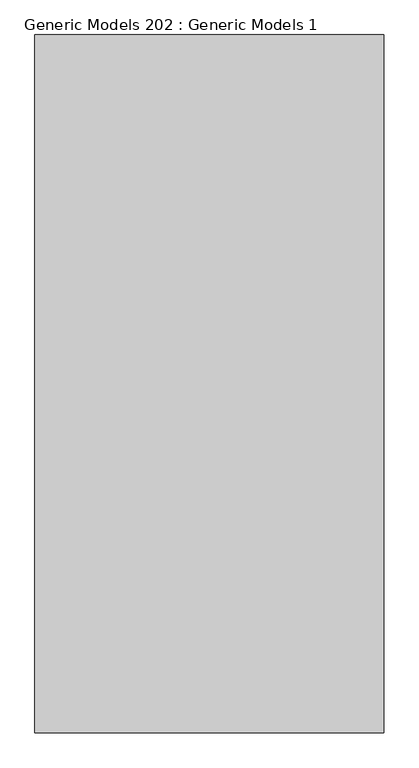
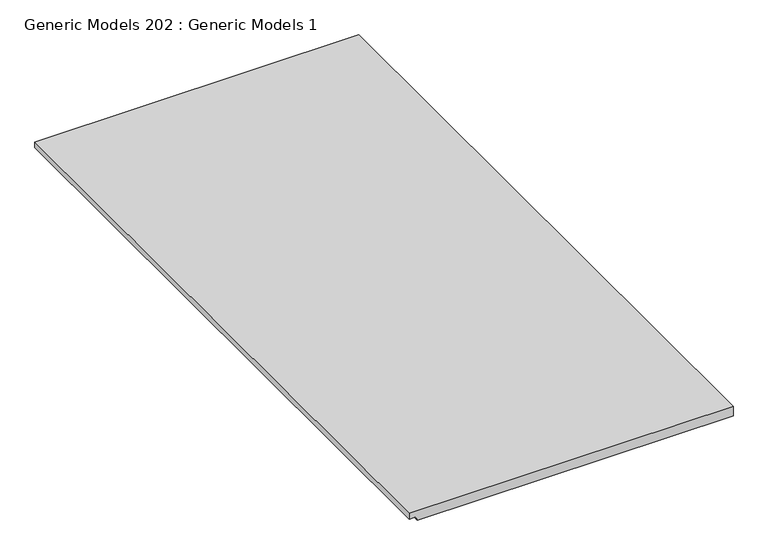
"""IFC4 building model written with IfcOpenShell, lengths in millimetres: proxy geometry, Generic Models 202 : Generic Models 1."""

import ifcopenshell
import ifcopenshell.guid

model = None  # the IFC model being written
_history = None  # IfcOwnerHistory: only IFC2X3 demands one
_inside = {}  # id of a spatial element -> (the spatial element, [elements in it])
_under = {}  # id of a project, library or spatial element -> (it, [spatial elements below it])
_declared = {}  # id of a project -> (the project, [libraries it declares])
_typed = {}  # id of a type object -> (the type object, [elements of that type])
_made_of = {}  # id of a material, layer set ... -> (it, [elements and type objects made of it])


def new_model(schema):
    """Start an empty IFC model of exactly this schema.

    Asked for "IFC4X3", IfcOpenShell would pick the latest addendum, in which some entities
    have other attributes; the version numbers below select the first issue.
    IFC2X3 requires an IfcOwnerHistory on every rooted entity: one is made here for all.
    """
    global model, _history
    if schema == "IFC4X3":
        model = ifcopenshell.file(schema_version=(4, 3, 0, 0))
    else:
        model = ifcopenshell.file(schema=schema)
    _inside.clear()
    _under.clear()
    _declared.clear()
    _typed.clear()
    _made_of.clear()
    _history = None
    if model.schema == "IFC2X3":
        org = make("IfcOrganization", Name="unknown")
        user = make(
            "IfcPersonAndOrganization",
            ThePerson=make("IfcPerson", FamilyName="unknown"),
            TheOrganization=org,
        )
        app = make(
            "IfcApplication",
            ApplicationDeveloper=org,
            Version="unknown",
            ApplicationFullName="unknown",
            ApplicationIdentifier="unknown",
        )
        _history = make(
            "IfcOwnerHistory",
            OwningUser=user,
            OwningApplication=app,
            ChangeAction="ADDED",
            CreationDate=0,
        )
    return model


def make(cls, **values):
    """One entity of the class cls with the attributes given. An attribute that is None is left unset."""
    return model.create_entity(
        cls, **{name: value for name, value in values.items() if value is not None}
    )


def rooted(cls, **values):
    """An entity with a GlobalId (a new one), such as an element, a storey or a relation."""
    return make(cls, GlobalId=ifcopenshell.guid.new(), OwnerHistory=_history, **values)


def si_unit(unit_type, name, prefix=None):
    """IfcSIUnit, for example si_unit("LENGTHUNIT", "METRE", prefix="MILLI")."""
    return make("IfcSIUnit", UnitType=unit_type, Prefix=prefix, Name=name)


def assignment(units):
    """IfcUnitAssignment: the units of a project."""
    return None if units is None else make("IfcUnitAssignment", Units=units)


def point(xyz):
    """IfcCartesianPoint."""
    return None if xyz is None else make("IfcCartesianPoint", Coordinates=xyz)


def direction(xyz):
    """IfcDirection."""
    return None if xyz is None else make("IfcDirection", DirectionRatios=xyz)


def frame(location, z_axis=None, x_axis=None):
    """IfcAxis2Placement3D, a coordinate frame: its origin and axes. An axis left out is left unset."""
    return make(
        "IfcAxis2Placement3D",
        Location=point(location),
        Axis=direction(z_axis),
        RefDirection=direction(x_axis),
    )


def origin():
    """The frame at (0, 0, 0) with its axes left unset."""
    return frame((0.0, 0.0, 0.0))


def place(relative_to, where):
    """IfcLocalPlacement: puts the frame where relative to a parent placement (None: the world)."""
    return make(
        "IfcLocalPlacement", PlacementRelTo=relative_to, RelativePlacement=where
    )


def context(
    kind, dimensions, precision=None, world=None, true_north=None, identifier=None
):
    """IfcGeometricRepresentationContext, for example the 3D "Model" context."""
    return make(
        "IfcGeometricRepresentationContext",
        ContextIdentifier=identifier,
        ContextType=kind,
        CoordinateSpaceDimension=dimensions,
        Precision=precision,
        WorldCoordinateSystem=world,
        TrueNorth=true_north,
    )


def project(units=None, contexts=None):
    """IfcProject with its units and contexts."""
    return rooted(
        "IfcProject",
        Name="project",
        RepresentationContexts=contexts,
        UnitsInContext=assignment(units),
    )


def spatial(cls, under=None, at=None, **own):
    """A site, building, storey or space (cls), placed at a placement, below another one or the project."""
    s = rooted(cls, ObjectPlacement=at, **own)
    if under is not None:
        _under.setdefault(under.id(), (under, []))[1].append(s)
    return s


def polyline(points):
    """IfcPolyline through the points."""
    return make("IfcPolyline", Points=[point(p) for p in points])


def outline(outer, holes=None, kind="AREA"):
    """IfcArbitraryClosedProfileDef: a profile drawn as a closed curve; with holes, ...WithVoids."""
    if holes is None:
        return make("IfcArbitraryClosedProfileDef", ProfileType=kind, OuterCurve=outer)
    return make(
        "IfcArbitraryProfileDefWithVoids",
        ProfileType=kind,
        OuterCurve=outer,
        InnerCurves=holes,
    )


def extrude(swept, where, along, depth):
    """IfcExtrudedAreaSolid: the profile swept, set in the frame where, extruded along a direction by depth."""
    return make(
        "IfcExtrudedAreaSolid",
        SweptArea=swept,
        Position=where,
        ExtrudedDirection=direction(along),
        Depth=depth,
    )


def shape(context_of_items, identifier, shape_type, items):
    """IfcShapeRepresentation: the items that make up one representation, for example the "Body"."""
    return make(
        "IfcShapeRepresentation",
        ContextOfItems=context_of_items,
        RepresentationIdentifier=identifier,
        RepresentationType=shape_type,
        Items=items,
    )


def source(mapping_origin, context_of_items, identifier, shape_type, items):
    """IfcRepresentationMap: a shape defined once, which mapped items show again and again."""
    return make(
        "IfcRepresentationMap",
        MappingOrigin=mapping_origin,
        MappedRepresentation=shape(context_of_items, identifier, shape_type, items),
    )


def transform(
    local_origin,
    x_axis=None,
    y_axis=None,
    z_axis=None,
    scale=None,
    scale2=None,
    scale3=None,
    uniform=True,
):
    """IfcCartesianTransformationOperator3D, or its non-uniform kind. x_axis, y_axis, z_axis: its Axis1, 2, 3."""
    if uniform:
        return make(
            "IfcCartesianTransformationOperator3D",
            Axis1=direction(x_axis),
            Axis2=direction(y_axis),
            LocalOrigin=point(local_origin),
            Scale=scale,
            Axis3=direction(z_axis),
        )
    return make(
        "IfcCartesianTransformationOperator3DnonUniform",
        Axis1=direction(x_axis),
        Axis2=direction(y_axis),
        LocalOrigin=point(local_origin),
        Scale=scale,
        Axis3=direction(z_axis),
        Scale2=scale2,
        Scale3=scale3,
    )


def mapped(mapping_source, mapping_target):
    """IfcMappedItem: shows the shape of a source again, moved by a transform."""
    return make(
        "IfcMappedItem", MappingSource=mapping_source, MappingTarget=mapping_target
    )


def made_of(thing, what):
    """Note that an element or type object is made of a material, layer set ...; save() writes the relation."""
    if what is not None:
        _made_of.setdefault(what.id(), (what, []))[1].append(thing)
    return thing


def element(
    cls,
    number,
    at=None,
    inside=None,
    cuts=None,
    type_object=None,
    material=None,
    context=None,
    identifier="Body",
    shape_type=None,
    held_by="IfcProductDefinitionShape",
    body=None,
    shapes=None,
    **own,
):
    """One element of the class cls, such as IfcWall. Its Tag is "e" and its number.

    at: its placement. inside: the storey or other place that contains it. cuts: it is an
    opening in that element (IfcRelVoidsElement). A single representation is given by context,
    identifier, shape_type and body (its items); several are given by shapes. held_by: the class
    of the entity that holds the representations. save() writes the other relations.
    """
    e = rooted(cls, Tag="e%d" % number, ObjectPlacement=at, **own)
    if body is not None:
        shapes = [shape(context, identifier, shape_type, body)]
    if shapes is not None:
        e.Representation = make(held_by, Representations=shapes)
    if inside is not None:
        _inside.setdefault(inside.id(), (inside, []))[1].append(e)
    if cuts is not None:
        rooted(
            "IfcRelVoidsElement", RelatingBuildingElement=cuts, RelatedOpeningElement=e
        )
    if type_object is not None:
        _typed.setdefault(type_object.id(), (type_object, []))[1].append(e)
    return made_of(e, material)


def aggregate(whole, parts):
    """IfcRelAggregates: a whole, such as a stair, and the parts it consists of."""
    return rooted("IfcRelAggregates", RelatingObject=whole, RelatedObjects=parts)


def save(model, path):
    """Write the relations noted so far, then the file.

    IfcRelAggregates (storeys below a building ...), IfcRelContainedInSpatialStructure (elements
    in a storey), IfcRelDefinesByType, IfcRelAssociatesMaterial and IfcRelDeclares: one each for
    every whole, place, type object, material and project.
    """
    for whole, parts in _under.values():
        aggregate(whole, parts)
    for where, things in _inside.values():
        rooted(
            "IfcRelContainedInSpatialStructure",
            RelatedElements=things,
            RelatingStructure=where,
        )
    for kind, things in _typed.values():
        rooted("IfcRelDefinesByType", RelatedObjects=things, RelatingType=kind)
    for what, things in _made_of.values():
        rooted("IfcRelAssociatesMaterial", RelatedObjects=things, RelatingMaterial=what)
    for by, libraries in _declared.values():
        rooted("IfcRelDeclares", RelatingContext=by, RelatedDefinitions=libraries)
    model.write(path)


def generic_models_202_generic_models_1_0ad20a8b(model_context):
    return source(origin(), model_context, "Body", "SweptSolid", [
        extrude(outline(polyline([(2253.330428, 49813.3451407), (2242.217928, 49813.3451407), (2242.217928, 49826.0451407), (2234.280428, 49828.9341545), (2234.280428, 50422.9451407), (2253.330428, 50422.9451407), (2253.330428, 49813.3451407)])), frame((0.0, 0.0, 0.0), z_axis=(0.0, 1.0, 0.0), x_axis=(0.0, 0.0, 1.0)), (0.0, 0.0, 1.0), 1219.2),
    ])


if __name__ == "__main__":
    model = new_model("IFC4")
    model_context = context("Model", 3, world=origin())
    ifc_project = project(units=[si_unit("LENGTHUNIT", "METRE", prefix="MILLI")], contexts=[model_context])
    site = spatial("IfcSite", under=ifc_project)
    building = spatial("IfcBuilding", under=site)
    placement = place(None, origin())
    generic_models_202_generic_models_1_shape = generic_models_202_generic_models_1_0ad20a8b(model_context)
    element("IfcBuildingElementProxy", 1, Name="Generic Models 202 : Generic Models 1", ObjectType="Generic Models 202 : Generic Models 1", at=placement, inside=building, context=model_context, shape_type="MappedRepresentation", body=[
        mapped(generic_models_202_generic_models_1_shape, transform((0.0, 0.0, 0.0), x_axis=(1.0, 0.0, 0.0), y_axis=(0.0, 1.0, 0.0), z_axis=(0.0, 0.0, 1.0))),
    ])
    save(model, "model.ifc")

# Revit data of these elements
# Element 1 (IfcBuildingElementProxy, "Generic Models 202 : Generic Models 1")
#   Materials on its faces: "CEILING AS SCHEDULED"
# Materials
#   "CEILING AS SCHEDULED": class "Generic", colour RGB 255 255 255, transparency 0, Cost = 0
